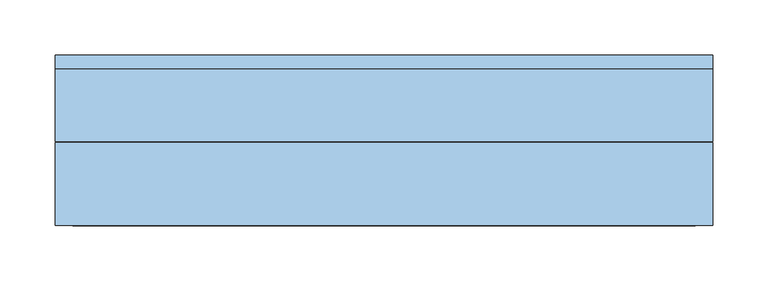
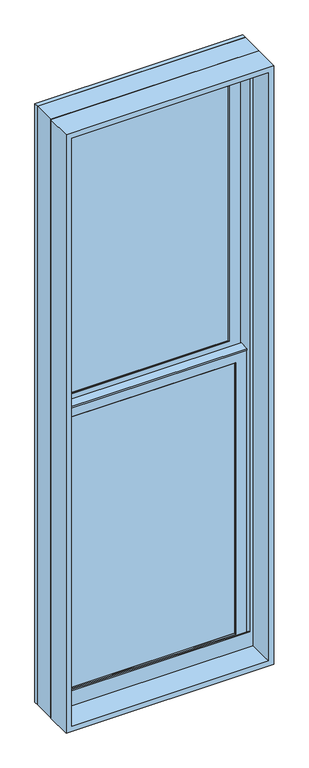
"""IFC4 building model written with IfcOpenShell, lengths in millimetres: window geometry, Window-Double_Hung-Marvin-Essential : ESDH2060."""

from ifc_helpers import new_model, si_unit, frame, origin, place, context, project, spatial, polyline, outline, extrude, faceted_brep, source, transform, mapped, element, save


def window_e668f755(model_context):
    return source(origin(), model_context, "Body", "SolidModel", [
        extrude(outline(polyline([(89.9583333, 20.6375), (89.9583333, 15.875), (70.9083333, 15.875), (70.9083333, 20.6375), (89.9583333, 20.6375)])), frame((0.0, 0.0, 679.45), z_axis=(0.0, 0.0, 1.0), x_axis=(1.0, 0.0, 0.0)), (0.0, 0.0, 1.0), 831.85),
        extrude(outline(polyline([(-70.9083333, 20.6375), (-70.9083333, 15.875), (-89.9583333, 15.875), (-89.9583333, 20.6375), (-70.9083333, 20.6375)])), frame((0.0, 0.0, 679.45), z_axis=(0.0, 0.0, 1.0), x_axis=(1.0, 0.0, 0.0)), (0.0, 0.0, 1.0), 831.85),
        extrude(outline(polyline([(241.3, 20.6375), (241.3, 15.875), (-241.3, 15.875), (-241.3, 20.6375), (241.3, 20.6375)])), frame((0.0, 0.0, 1085.85), z_axis=(0.0, 0.0, 1.0), x_axis=(1.0, 0.0, 0.0)), (0.0, 0.0, 1.0), 19.05),
        extrude(outline(polyline([(-89.9583333, 46.83125), (-89.9583333, 51.59375), (-70.9083333, 51.59375), (-70.9083333, 46.83125), (-89.9583333, 46.83125)])), frame((0.0, 0.0, 1549.4), z_axis=(0.0, 0.0, 1.0), x_axis=(1.0, 0.0, 0.0)), (0.0, 0.0, 1.0), 831.85),
        extrude(outline(polyline([(70.9083333, 46.83125), (70.9083333, 51.59375), (89.9583333, 51.59375), (89.9583333, 46.83125), (70.9083333, 46.83125)])), frame((0.0, 0.0, 1549.4), z_axis=(0.0, 0.0, 1.0), x_axis=(1.0, 0.0, 0.0)), (0.0, 0.0, 1.0), 831.85),
        extrude(outline(polyline([(-241.3, 46.83125), (-241.3, 51.59375), (241.3, 51.59375), (241.3, 46.83125), (-241.3, 46.83125)])), frame((0.0, 0.0, 1955.8), z_axis=(0.0, 0.0, 1.0), x_axis=(1.0, 0.0, 0.0)), (0.0, 0.0, 1.0), 19.05),
        extrude(outline(polyline([(89.9583333, 20.6375), (70.9083333, 20.6375), (70.9083333, 25.4), (89.9583333, 25.4), (89.9583333, 20.6375)])), frame((0.0, 0.0, 679.45), z_axis=(0.0, 0.0, 1.0), x_axis=(1.0, 0.0, 0.0)), (0.0, 0.0, 1.0), 831.85),
        extrude(outline(polyline([(-70.9083333, 20.6375), (-89.9583333, 20.6375), (-89.9583333, 25.4), (-70.9083333, 25.4), (-70.9083333, 20.6375)])), frame((0.0, 0.0, 679.45), z_axis=(0.0, 0.0, 1.0), x_axis=(1.0, 0.0, 0.0)), (0.0, 0.0, 1.0), 831.85),
        extrude(outline(polyline([(241.3, 20.6375), (-241.3, 20.6375), (-241.3, 25.4), (241.3, 25.4), (241.3, 20.6375)])), frame((0.0, 0.0, 1085.85), z_axis=(0.0, 0.0, 1.0), x_axis=(1.0, 0.0, 0.0)), (0.0, 0.0, 1.0), 19.05),
        extrude(outline(polyline([(-89.9583333, 56.35625), (-70.9083333, 56.35625), (-70.9083333, 51.59375), (-89.9583333, 51.59375), (-89.9583333, 56.35625)])), frame((0.0, 0.0, 1549.4), z_axis=(0.0, 0.0, 1.0), x_axis=(1.0, 0.0, 0.0)), (0.0, 0.0, 1.0), 831.85),
        extrude(outline(polyline([(70.9083333, 56.35625), (89.9583333, 56.35625), (89.9583333, 51.59375), (70.9083333, 51.59375), (70.9083333, 56.35625)])), frame((0.0, 0.0, 1549.4), z_axis=(0.0, 0.0, 1.0), x_axis=(1.0, 0.0, 0.0)), (0.0, 0.0, 1.0), 831.85),
        extrude(outline(polyline([(-241.3, 56.35625), (241.3, 56.35625), (241.3, 51.59375), (-241.3, 51.59375), (-241.3, 56.35625)])), frame((0.0, 0.0, 1955.8), z_axis=(0.0, 0.0, 1.0), x_axis=(1.0, 0.0, 0.0)), (0.0, 0.0, 1.0), 19.05),
        faceted_brep([(-268.2875, 5.6780605, 1541.3351748), (-268.2875, 5.6780605, 1536.7), (268.2875, 5.6780605, 1536.7), (268.2875, 5.6780605, 1541.3351748), (-268.2875, 34.8118605, 1541.3351748), (268.2875, 34.8118605, 1541.3351748), (268.2875, 34.8118605, 1536.7), (-268.2875, 34.8118605, 1536.7), (-268.2875, 30.1625, 1536.7), (-268.2875, 30.1625, 652.4625), (-268.2875, 8.9241104, 652.4625), (-268.2875, 8.9241104, 1536.7), (268.2875, 8.9241104, 1536.7), (268.2875, 30.1625, 1536.7), (268.2875, 8.9241104, 652.4625), (268.2875, 30.1625, 652.4625), (-252.4034752, 11.90625, 1522.4034752), (-252.4034752, 30.1625, 1522.4034752), (252.4034752, 30.1625, 1522.4034752), (252.4034752, 11.90625, 1522.4034752), (-235.74375, 10.4662439, 1505.74375), (-235.74375, 11.90625, 1505.74375), (235.74375, 11.90625, 1505.74375), (235.74375, 10.4662439, 1505.74375), (237.2858834, 8.9241104, 1507.2858834), (-237.2858834, 8.9241104, 1507.2858834), (252.4034752, 30.1625, 668.3465248), (252.4034752, 11.90625, 668.3465248), (235.74375, 11.90625, 685.00625), (235.74375, 10.4662439, 685.00625), (237.2858834, 8.9241104, 683.4641166), (-252.4034752, 30.1625, 668.3465248), (-252.4034752, 11.90625, 668.3465248), (-235.74375, 11.90625, 685.00625), (-235.74375, 10.4662439, 685.00625), (-237.2858834, 8.9241104, 683.4641166)], [[[0, 1, 2, 3]], [[4, 5, 6, 7]], [[1, 0, 4, 7, 8, 9, 10, 11]], [[2, 1, 11, 12]], [[7, 6, 13, 8]], [[3, 2, 12, 14, 15, 13, 6, 5]], [[0, 3, 5, 4]], [[16, 17, 18, 19]], [[20, 21, 22, 23]], [[20, 23, 24, 25]], [[19, 18, 26, 27]], [[23, 22, 28, 29]], [[24, 23, 29, 30]], [[27, 26, 31, 32]], [[29, 28, 33, 34]], [[30, 29, 34, 35]], [[15, 14, 10, 9]], [[15, 9, 8, 13], [18, 17, 31, 26]], [[17, 16, 32, 31]], [[16, 19, 27, 32], [22, 21, 33, 28]], [[21, 20, 34, 33]], [[20, 25, 35, 34]], [[10, 14, 12, 11], [25, 24, 30, 35]]]),
        extrude(outline(polyline([(38.5955581, 1522.4125), (33.5778968, 1522.4125), (33.5778968, 1524.0), (39.9405976, 1524.0), (39.9405976, 1522.4125), (61.515625, 1522.4125), (47.6307501, 1519.0975159), (38.5955581, 1519.0975159), (38.5955581, 1522.4125)])), frame((-268.2875, 0.0, 0.0), z_axis=(1.0, 0.0, 0.0), x_axis=(0.0, 1.0, 0.0)), (0.0, 0.0, 1.0), 536.575),
        faceted_brep([(298.45, 0.0, 622.3), (298.45, 0.0, 2438.4), (-298.45, 0.0, 2438.4), (-298.45, 0.0, 622.3), (272.25625, 0.0, 683.41875), (-272.25625, 0.0, 683.41875), (-272.25625, 0.0, 2412.20625), (272.25625, 0.0, 2412.20625), (272.25625, 3.96875, 622.3), (-272.25625, 3.96875, 622.3), (-272.25625, 3.96875, 683.41875), (272.25625, 3.96875, 683.41875), (-298.45, 65.6828125, 622.3), (-272.25625, 65.6828125, 622.3), (272.25625, 65.6828125, 622.3), (298.45, 65.6828125, 622.3), (-298.45, 65.6828125, 2438.4), (298.45, 65.6828125, 2438.4), (272.25625, 65.6828125, 2412.20625), (-272.25625, 65.6828125, 2412.20625)], [[[0, 1, 2, 3], [4, 5, 6, 7]], [[8, 9, 10, 11]], [[5, 4, 11, 10]], [[0, 3, 12, 13, 9, 8, 14, 15]], [[13, 12, 16, 17, 15, 14, 18, 19]], [[13, 19, 6, 5, 10, 9]], [[7, 6, 19, 18]], [[18, 14, 8, 11, 4, 7]], [[1, 0, 15, 17]], [[2, 1, 17, 16]], [[3, 2, 16, 12]]]),
        faceted_brep([(272.25625, 30.1625, 1530.35), (270.66875, 30.1625, 1530.35), (270.66875, 30.1625, 646.6544613), (272.25625, 30.1625, 646.6544613), (-270.66875, 30.1625, 1530.35), (-272.25625, 30.1625, 1530.35), (-272.25625, 30.1625, 646.6544613), (-270.66875, 30.1625, 646.6544613), (270.66875, 63.5, 1530.35), (272.25625, 63.5, 1530.35), (272.25625, 63.5, 640.1743077), (270.66875, 63.5, 640.1743077), (-272.25625, 63.5, 1530.35), (-270.66875, 63.5, 1530.35), (-270.66875, 63.5, 640.1743077), (-272.25625, 63.5, 640.1743077), (283.5108932, 3.96875, 651.7460105), (283.5108932, 3.96875, 622.3), (283.5108932, 65.6828125, 622.3), (283.5108932, 65.6828125, 639.750012), (-283.5108932, 3.96875, 622.3), (-283.5108932, 3.96875, 651.7460105), (-283.5108932, 65.6828125, 639.750012), (-283.5108932, 65.6828125, 622.3), (283.5108932, 78.58125, 637.2428097), (-283.5108932, 78.58125, 637.2428097), (-281.4971252, 68.2348864, 639.2539391), (-263.53135, 68.2348864, 639.2539391), (-263.53135, 65.6828125, 639.750012), (263.53135, 65.6828125, 639.750012), (263.53135, 68.2348864, 639.2539391), (281.4971252, 68.2348864, 639.2539391), (-298.45, 65.6828125, 622.3), (-298.45, 78.5948249, 622.3), (298.45, 78.5948249, 622.3), (298.45, 65.6828125, 622.3), (-298.45, 78.58125, 2438.4), (298.45, 78.58125, 2438.4), (283.5108932, 78.58125, 2423.4608932), (-283.5108932, 78.58125, 2423.4608932), (-298.45, 65.6828125, 2438.4), (-281.4971252, 68.2348864, 2421.4471252), (281.4971252, 68.2348864, 2421.4471252), (263.53135, 68.2348864, 2403.48135), (-263.53135, 68.2348864, 2403.48135), (-263.53135, 65.6828125, 2403.48135), (263.53135, 65.6828125, 2403.48135), (298.45, 65.6828125, 2438.4)], [[[0, 1, 2, 3]], [[4, 5, 6, 7]], [[8, 9, 10, 11]], [[12, 13, 14, 15]], [[1, 8, 11, 2]], [[9, 0, 3, 10]], [[1, 0, 9, 8]], [[5, 4, 13, 12]], [[5, 12, 15, 6]], [[13, 4, 7, 14]], [[16, 17, 18, 19]], [[20, 21, 22, 23]], [[24, 25, 26, 27, 28, 22, 21, 16, 19, 29, 30, 31], [3, 2, 11, 10], [7, 6, 15, 14]], [[17, 16, 21, 20]], [[17, 20, 23, 32, 33, 34, 35, 18]], [[34, 33, 36, 37], [25, 24, 38, 39]], [[33, 32, 40, 36]], [[39, 41, 26, 25]], [[41, 42, 31, 30, 43, 44, 27, 26]], [[44, 45, 28, 27]], [[40, 32, 23, 22, 28, 45, 46, 29, 19, 18, 35, 47]], [[36, 40, 47, 37]], [[39, 38, 42, 41]], [[44, 43, 46, 45]], [[34, 37, 47, 35]], [[42, 38, 24, 31]], [[46, 43, 30, 29]]]),
        extrude(outline(polyline([(248.44375, 11.90625), (-248.44375, 11.90625), (-248.44375, 15.08125), (248.44375, 15.08125), (248.44375, 11.90625)])), frame((0.0, 0.0, 672.30625), z_axis=(0.0, 0.0, 1.0), x_axis=(1.0, 0.0, 0.0)), (0.0, 0.0, 1.0), 846.1375),
        extrude(outline(polyline([(248.44375, 42.8625), (-248.44375, 42.8625), (-248.44375, 46.0375), (248.44375, 46.0375), (248.44375, 42.8625)])), frame((0.0, 0.0, 1542.25625), z_axis=(0.0, 0.0, 1.0), x_axis=(1.0, 0.0, 0.0)), (0.0, 0.0, 1.0), 846.1375),
        faceted_brep([(-235.74375, 31.194477, 1505.74375), (-237.2858834, 32.7366104, 1507.2858834), (237.2858834, 32.7366104, 1507.2858834), (235.74375, 31.194477, 1505.74375), (-235.74375, 30.1625, 1505.74375), (235.74375, 30.1625, 1505.74375), (-268.2875, 32.7366104, 1538.2875), (-268.2875, 30.1625, 1538.2875), (268.2875, 30.1625, 1538.2875), (268.2875, 32.7366104, 1538.2875), (237.2858834, 32.7366104, 683.4641166), (235.74375, 31.194477, 685.00625), (235.74375, 30.1625, 685.00625), (268.2875, 30.1625, 652.4625), (268.2875, 32.7366104, 652.4625), (-237.2858834, 32.7366104, 683.4641166), (-235.74375, 31.194477, 685.00625), (-235.74375, 30.1625, 685.00625), (-268.2875, 30.1625, 652.4625), (-268.2875, 32.7366104, 652.4625)], [[[0, 1, 2, 3]], [[4, 0, 3, 5]], [[6, 7, 8, 9]], [[3, 2, 10, 11]], [[5, 3, 11, 12]], [[9, 8, 13, 14]], [[11, 10, 15, 16]], [[12, 11, 16, 17]], [[14, 13, 18, 19]], [[9, 14, 19, 6], [1, 15, 10, 2]], [[16, 15, 1, 0]], [[17, 16, 0, 4]], [[7, 18, 13, 8], [5, 12, 17, 4]], [[19, 18, 7, 6]]]),
        faceted_brep([(-252.4034752, 42.8625, 2392.3534752), (-252.4034752, 61.11875, 2392.3534752), (252.4034752, 61.11875, 2392.3534752), (252.4034752, 42.8625, 2392.3534752), (-235.74375, 41.4224939, 2375.69375), (-235.74375, 42.8625, 2375.69375), (235.74375, 42.8625, 2375.69375), (235.74375, 41.4224939, 2375.69375), (-237.2858834, 39.8803604, 2377.2358834), (237.2858834, 39.8803604, 2377.2358834), (-268.2875, 61.11875, 2408.2375), (-268.2875, 39.8803604, 2408.2375), (268.2875, 39.8803604, 2408.2375), (268.2875, 61.11875, 2408.2375), (252.4034752, 61.11875, 1538.2965248), (252.4034752, 42.8625, 1538.2965248), (235.74375, 42.8625, 1554.95625), (235.74375, 41.4224939, 1554.95625), (237.2858834, 39.8803604, 1553.4141166), (268.2875, 39.8803604, 1522.4125), (268.2875, 61.11875, 1522.4125), (-252.4034752, 61.11875, 1538.2965248), (-252.4034752, 42.8625, 1538.2965248), (-235.74375, 42.8625, 1554.95625), (-235.74375, 41.4224939, 1554.95625), (-237.2858834, 39.8803604, 1553.4141166), (-268.2875, 39.8803604, 1522.4125), (-268.2875, 61.11875, 1522.4125)], [[[0, 1, 2, 3]], [[4, 5, 6, 7]], [[8, 4, 7, 9]], [[10, 11, 12, 13]], [[3, 2, 14, 15]], [[7, 6, 16, 17]], [[9, 7, 17, 18]], [[13, 12, 19, 20]], [[15, 14, 21, 22]], [[17, 16, 23, 24]], [[18, 17, 24, 25]], [[20, 19, 26, 27]], [[13, 20, 27, 10], [1, 21, 14, 2]], [[22, 21, 1, 0]], [[3, 15, 22, 0], [5, 23, 16, 6]], [[24, 23, 5, 4]], [[25, 24, 4, 8]], [[11, 26, 19, 12], [9, 18, 25, 8]], [[27, 26, 11, 10]]]),
        faceted_brep([(-268.2875, 61.11875, 1522.4125), (-268.2875, 63.6928604, 1522.4125), (268.2875, 63.6928604, 1522.4125), (268.2875, 61.11875, 1522.4125), (-235.74375, 62.150727, 1554.95625), (-235.74375, 61.11875, 1554.95625), (235.74375, 61.11875, 1554.95625), (235.74375, 62.150727, 1554.95625), (-237.2858834, 63.6928604, 1553.4141166), (237.2858834, 63.6928604, 1553.4141166), (268.2875, 63.6928604, 2408.2375), (268.2875, 61.11875, 2408.2375), (235.74375, 61.11875, 2375.69375), (235.74375, 62.150727, 2375.69375), (237.2858834, 63.6928604, 2377.2358834), (-268.2875, 63.6928604, 2408.2375), (-268.2875, 61.11875, 2408.2375), (-235.74375, 61.11875, 2375.69375), (-235.74375, 62.150727, 2375.69375), (-237.2858834, 63.6928604, 2377.2358834)], [[[0, 1, 2, 3]], [[4, 5, 6, 7]], [[8, 4, 7, 9]], [[3, 2, 10, 11]], [[7, 6, 12, 13]], [[9, 7, 13, 14]], [[11, 10, 15, 16]], [[13, 12, 17, 18]], [[14, 13, 18, 19]], [[16, 15, 1, 0]], [[3, 11, 16, 0], [5, 17, 12, 6]], [[18, 17, 5, 4]], [[19, 18, 4, 8]], [[1, 15, 10, 2], [9, 14, 19, 8]]]),
        extrude(outline(polyline([(248.44375, 26.19375), (-248.44375, 26.19375), (-248.44375, 30.1625), (248.44375, 30.1625), (248.44375, 26.19375)])), frame((0.0, 0.0, 672.30625), z_axis=(0.0, 0.0, 1.0), x_axis=(1.0, 0.0, 0.0)), (0.0, 0.0, 1.0), 846.1375),
        extrude(outline(polyline([(248.44375, 57.15), (-248.44375, 57.15), (-248.44375, 61.11875), (248.44375, 61.11875), (248.44375, 57.15)])), frame((0.0, 0.0, 1542.25625), z_axis=(0.0, 0.0, 1.0), x_axis=(1.0, 0.0, 0.0)), (0.0, 0.0, 1.0), 846.1375),
        extrude(outline(polyline([(2438.4, 298.45), (2438.4, -298.45), (622.3, -298.45), (622.3, 298.45), (2438.4, 298.45)]), holes=[polyline([(2422.525, 282.575), (638.175, 282.575), (638.175, -282.575), (2422.525, -282.575), (2422.525, 282.575)])]), frame((0.0, -76.2, 0.0), z_axis=(0.0, 1.0, 0.0), x_axis=(0.0, 0.0, 1.0)), (0.0, 0.0, 1.0), 75.40625),
    ])


if __name__ == "__main__":
    model = new_model("IFC4")
    model_context = context("Model", 3, world=origin())
    ifc_project = project(units=[si_unit("LENGTHUNIT", "METRE", prefix="MILLI")], contexts=[model_context])
    site = spatial("IfcSite", under=ifc_project)
    building = spatial("IfcBuilding", under=site)
    placement = place(None, origin())
    window_shape = window_e668f755(model_context)
    element("IfcWindow", 1, ObjectType="Window-Double_Hung-Marvin-Essential : ESDH2060", at=placement, inside=building, context=model_context, shape_type="MappedRepresentation", body=[
        mapped(window_shape, transform((0.0, 0.0, 0.0), x_axis=(1.0, 0.0, 0.0), y_axis=(0.0, 1.0, 0.0), z_axis=(0.0, 0.0, 1.0))),
    ])
    save(model, "model.ifc")

# Revit data of these elements
# Type "Window-Double_Hung-Marvin-Essential : ESDH2060"
#   Type Mark = "76"
#   Window Type = "Essential Double Hung"
#   Product data url = "https://bimobject.com/marvin-windows-and-doors/product/marvin-dhwau"
#   Product Guid = "c4a96547-874c-4385-91dc-a058adc19d98"
#   Frame = "All Ultrex"
#   Egress Window = "No"
#   URL = "www.marvin.com"
#   Model = "ESDH2060"
#   Manufacturer = "Marvin Windows and Doors"
#   Label Egress = ""
#   Glass Type = "IG Low E II with Argon"
#   Design Pressure = "DP40"
#   Description = "2472 DBHG"
#   Analytic Construction = "<None>"
#   Prairie Corner Width = 0' - 4"
#   Prairie Corner Height = 0' - 4"
#   Egress Width = 1' - 8 9/16"
#   Egress Height = 2' - 7 27/128"
#   Rough Width = 2' - 0"
#   Rough Height = 6' - 0"
#   Nominal Width = 2' - 0"
#   Nominal Height = 6' - 0"
#   Inset to Installation Flange [instance default] = 0' - 1"
#   Height = 5' - 11 1/2"
#   Egress Area = 4.45677 SF
#   Default Head Height = 8' - 0"
#   Width = 1' - 11 1/2"
#   Daylight Area = 8.33057 SF
#   DLO Width = 1' - 6 9/16"
#   DLO Height = 2' - 8 5/16"
#   Muntins Top Sash = yes
#   Lites Wide Top Sash = 3
#   Lites Wide Bottom Sash = 3
#   Lites High Top Sash = 2
#   Lites High Bottom Sash = 2
#   Lite Cut Prairie 9 = no
#   Lite Cut HV Grid = yes
#   Muntins Bottom Sash = yes
#   Label Visibility = no
#   Jamb Extension Visibility = yes
#   Edition number = 1
#   Interior Material = Ultrex-Marvin-Stonewhite
#   Glazing Material = Glass-Marvin-IG Low E II with Argon
#   Cladding Material = Ultrex-Marvin-Pebblegray
#   Wall Closure = (empty or 0)
#   Assembly Code = ""
# Element 1 (IfcWindow, "Window-Double_Hung-Marvin-Essential : ESDH2060")
#   Materials on its faces: "Ultrex-Marvin-Pebblegray", "Ultrex-Marvin-Stonewhite", "Glass-Marvin-IG Low E II with Argon"
# Materials
#   "Ultrex-Marvin-Stonewhite": class "Paint", colour RGB 250 251 245, transparency 0
#   "Glass-Marvin-IG Low E II with Argon": class "Glass", colour RGB 0 128 192, transparency 0.85
#   "Ultrex-Marvin-Pebblegray": class "Paint", colour RGB 189 185 173, transparency 0
